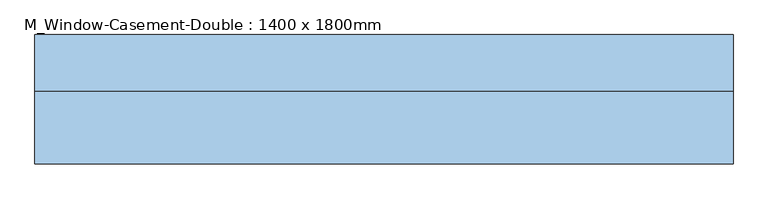
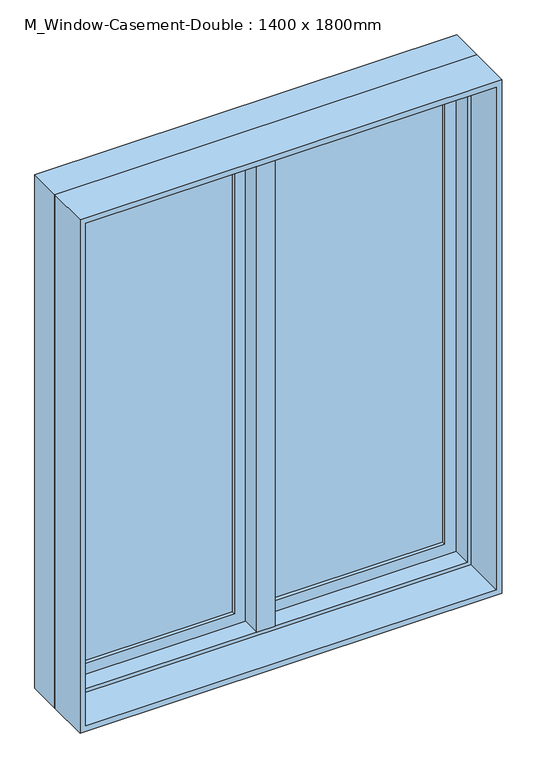
"""IFC4 building model written with IfcOpenShell, lengths in millimetres: window geometry, M_Window-Casement-Double : 1400 x 1800mm."""

from ifc_helpers import new_model, si_unit, frame, origin, place, context, project, spatial, polyline, outline, extrude, faceted_brep, source, transform, mapped, element, save


def m_window_casement_double_1400_x_1800mm_e3405f7f(model_context):
    return source(origin(), model_context, "Body", "SolidModel", [
        faceted_brep([(9.525, 139.05, 2687.3), (-9.525, 139.05, 2687.3), (-9.525, 88.25, 2687.3), (9.525, 88.25, 2687.3), (9.525, 139.05, 912.7), (9.525, 88.25, 912.7), (-9.525, 88.25, 912.7), (-9.525, 139.05, 912.7), (-9.525, 88.25, 931.75), (-9.525, 88.25, 2668.25), (-30.1625, 88.25, 931.75), (-30.1625, 88.25, 2668.25), (-30.1625, 24.75, 931.75), (-30.1625, 24.75, 2668.25), (30.1625, 24.75, 931.75), (30.1625, 24.75, 2668.25), (30.1625, 88.25, 931.75), (30.1625, 88.25, 2668.25), (9.525, 88.25, 931.75), (9.525, 88.25, 2668.25)], [[[0, 1, 2, 3]], [[4, 5, 6, 7]], [[1, 0, 4, 7]], [[2, 1, 7, 6, 8, 9]], [[9, 8, 10, 11]], [[11, 10, 12, 13]], [[13, 12, 14, 15]], [[15, 14, 16, 17]], [[17, 16, 18, 19]], [[0, 3, 19, 18, 5, 4]], [[18, 8, 6, 5]], [[9, 19, 3, 2]], [[8, 18, 16, 14, 12, 10]], [[19, 9, 11, 13, 15, 17]]]),
        extrude(outline(polyline([(-66.675, 120.0), (-66.675, 113.65), (-630.15, 113.65), (-630.15, 120.0), (-66.675, 120.0)])), frame((0.0, 0.0, 969.85), z_axis=(0.0, 0.0, 1.0), x_axis=(1.0, 0.0, 0.0)), (0.0, 0.0, 1.0), 1660.3),
        extrude(outline(polyline([(-630.15, 100.95), (-630.15, 107.3), (-66.675, 107.3), (-66.675, 100.95), (-630.15, 100.95)])), frame((0.0, 0.0, 969.85), z_axis=(0.0, 0.0, 1.0), x_axis=(1.0, 0.0, 0.0)), (0.0, 0.0, 1.0), 1660.3),
        extrude(outline(polyline([(630.15, 120.0), (630.15, 113.65), (66.675, 113.65), (66.675, 120.0), (630.15, 120.0)])), frame((0.0, 0.0, 969.85), z_axis=(0.0, 0.0, 1.0), x_axis=(1.0, 0.0, 0.0)), (0.0, 0.0, 1.0), 1660.3),
        extrude(outline(polyline([(66.675, 100.95), (66.675, 107.3), (630.15, 107.3), (630.15, 100.95), (66.675, 100.95)])), frame((0.0, 0.0, 969.85), z_axis=(0.0, 0.0, 1.0), x_axis=(1.0, 0.0, 0.0)), (0.0, 0.0, 1.0), 1660.3),
        extrude(outline(polyline([(2687.3, -687.3), (912.7, -687.3), (912.7, -9.525), (2687.3, -9.525), (2687.3, -687.3)]), holes=[polyline([(2630.15, -66.675), (969.85, -66.675), (969.85, -630.15), (2630.15, -630.15), (2630.15, -66.675)])]), frame((0.0, 88.25, 0.0), z_axis=(0.0, 1.0, 0.0), x_axis=(0.0, 0.0, 1.0)), (0.0, 0.0, 1.0), 44.45),
        extrude(outline(polyline([(912.7, 687.3), (2687.3, 687.3), (2687.3, 9.525), (912.7, 9.525), (912.7, 687.3)]), holes=[polyline([(969.85, 66.675), (2630.15, 66.675), (2630.15, 630.15), (969.85, 630.15), (969.85, 66.675)])]), frame((0.0, 88.25, 0.0), z_axis=(0.0, 1.0, 0.0), x_axis=(0.0, 0.0, 1.0)), (0.0, 0.0, 1.0), 44.45),
        extrude(outline(polyline([(2700.0, -700.0), (900.0, -700.0), (900.0, 700.0), (2700.0, 700.0), (2700.0, -700.0)]), holes=[polyline([(2680.95, 680.95), (919.05, 680.95), (919.05, -680.95), (2680.95, -680.95), (2680.95, 680.95)])]), frame((0.0, -120.0, 0.0), z_axis=(0.0, 1.0, 0.0), x_axis=(0.0, 0.0, 1.0)), (0.0, 0.0, 1.0), 144.75),
        faceted_brep([(668.25, 88.25, 2668.25), (668.25, 24.75, 2668.25), (-668.25, 24.75, 2668.25), (-668.25, 88.25, 2668.25), (687.3, 139.05, 2687.3), (687.3, 88.25, 2687.3), (-687.3, 88.25, 2687.3), (-687.3, 139.05, 2687.3), (700.0, 24.75, 2700.0), (700.0, 139.05, 2700.0), (-700.0, 139.05, 2700.0), (-700.0, 24.75, 2700.0), (-668.25, 24.75, 931.75), (-668.25, 88.25, 931.75), (-687.3, 88.25, 912.7), (-687.3, 139.05, 912.7), (-700.0, 139.05, 900.0), (-700.0, 24.75, 900.0), (668.25, 24.75, 931.75), (668.25, 88.25, 931.75), (687.3, 88.25, 912.7), (687.3, 139.05, 912.7), (700.0, 139.05, 900.0), (700.0, 24.75, 900.0)], [[[0, 1, 2, 3]], [[4, 5, 6, 7]], [[8, 9, 10, 11]], [[3, 2, 12, 13]], [[7, 6, 14, 15]], [[11, 10, 16, 17]], [[13, 12, 18, 19]], [[15, 14, 20, 21]], [[17, 16, 22, 23]], [[11, 17, 23, 8], [1, 18, 12, 2]], [[19, 18, 1, 0]], [[5, 20, 14, 6], [3, 13, 19, 0]], [[21, 20, 5, 4]], [[23, 22, 9, 8]], [[9, 22, 16, 10], [7, 15, 21, 4]]]),
    ])


if __name__ == "__main__":
    model = new_model("IFC4")
    model_context = context("Model", 3, world=origin())
    ifc_project = project(units=[si_unit("LENGTHUNIT", "METRE", prefix="MILLI")], contexts=[model_context])
    site = spatial("IfcSite", under=ifc_project)
    building = spatial("IfcBuilding", under=site)
    placement = place(None, origin())
    m_window_casement_double_1400_x_1800mm_shape = m_window_casement_double_1400_x_1800mm_e3405f7f(model_context)
    element("IfcWindow", 1, ObjectType="M_Window-Casement-Double : 1400 x 1800mm", at=placement, inside=building, context=model_context, shape_type="MappedRepresentation", body=[
        mapped(m_window_casement_double_1400_x_1800mm_shape, transform((0.0, 0.0, 0.0), x_axis=(1.0, 0.0, 0.0), y_axis=(0.0, 1.0, 0.0), z_axis=(0.0, 0.0, 1.0))),
    ])
    save(model, "model.ifc")

# Revit data of these elements
# Type "M_Window-Casement-Double : 1400 x 1800mm"
#   Type Mark = "26"
#   Fire Rating = "0.5h"
#   Assembly Code = "B2020100"
#   Analytic Construction = "Double glazing - domestic"
#   Frame Extension [instance default] = 0.635 cm
#   Window Inset [instance default] = 0 cm
#   Wall Thickness [instance default] = 15 cm
#   Interior Wall Closure [instance default] = 5.475 cm
#   Half Width = 70 cm
#   Visual Light Transmittance = 0.81
#   Thermal Resistance (R) = 0.319569 (m²·K)/W
#   Solar Heat Gain Coefficient = 0.76
#   Rough Width = 141.5 cm
#   Rough Height = 181.5 cm
#   Height = 180 cm
#   Heat Transfer Coefficient (U) = 3.12929 W/(m²·K)
#   Exterior Wall Closure [instance default] = 3.18 cm
#   Extension Jamb [instance default] = 5.475 cm
#   Default Sill Height = 90 cm
#   Width = 140 cm
#   Muntin Visibility = yes
#   Interior Trim Visibility [instance default] = yes
#   Exterior Trim Visibility [instance default] = yes
#   Extension Jamb Visibility [instance default] = yes
#   Interior Trim Material = Wood - Stained
#   Muntin Pattern = M_Muntin Pattern_2x2 : M_Muntin Pattern_2x2
#   Interior Trim = M_Trim-Window-Interior-Flat : Picture Frame
#   Interior Frame Material = Wood - Stained
#   Glass Panel Material = Glass
#   Exterior Trim Material = Clad - White
#   Exterior Trim = M_Trim-Window-Exterior-Flat : with Sill
#   Exterior Frame Material = Clad - White
#   Wall Closure = (empty or 0)
# Element 1 (IfcWindow, "M_Window-Casement-Double : 1400 x 1800mm")
#   Wall Thickness = 24 cm
#   Extension Jamb = 14.475 cm
#   Materials on its faces: "Wood - Stained", "Glass", "Clad - White"
# Materials
#   "Wood - Stained": class "Wood", colour RGB 224 178 126, transparency 0, Cost = 0
#   "Glass": class "Glass", colour RGB 0 128 192, transparency 0.9, Description = "Soda Lime Glass", Cost = 0
#   "Clad - White": class "Wood", colour RGB 242 242 238, transparency 0, Cost = 0
